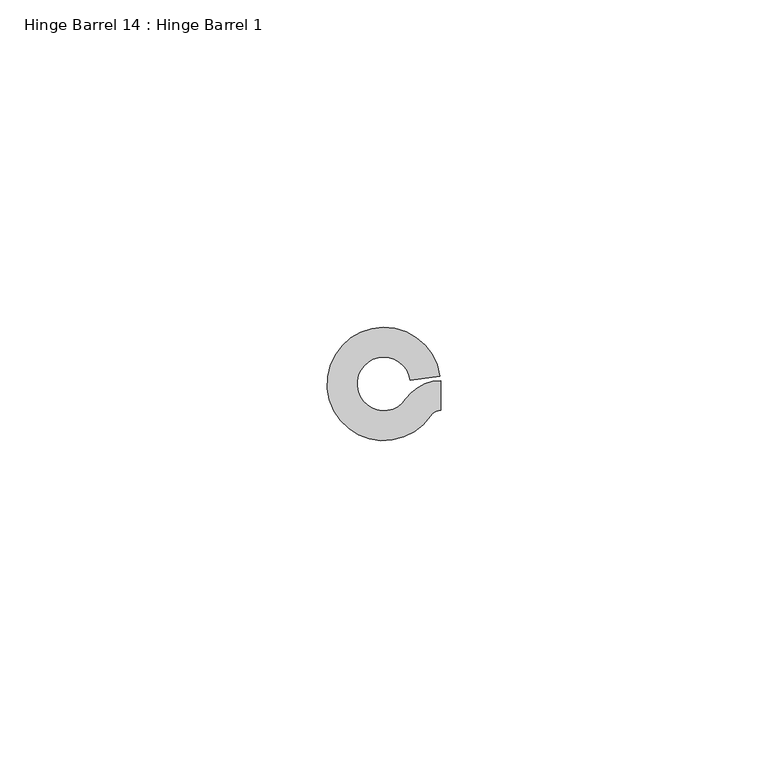
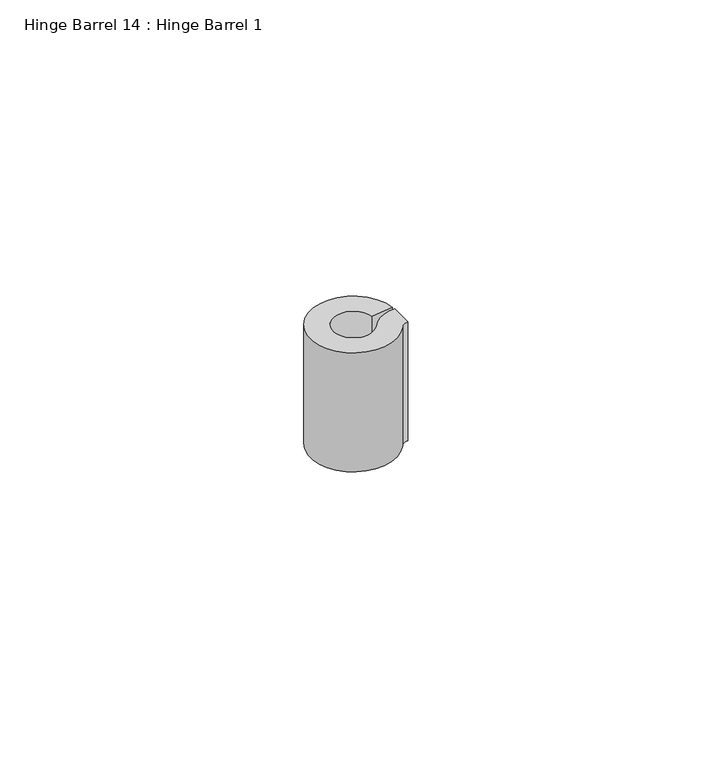
"""IFC4 building model written with IfcOpenShell, lengths in millimetres: proxy geometry, Hinge Barrel 14 : Hinge Barrel 1."""

from ifc_helpers import new_model, si_unit, point, frame, frame_2d, origin, place, context, project, spatial, polyline, circle_curve, trimmed, segment, composite_curve, outline, extrude, source, transform, mapped, element, save


def hinge_barrel_14_hinge_barrel_1_75b3f5ff(model_context):
    return source(origin(), model_context, "Body", "SweptSolid", [
        extrude(outline(composite_curve([segment(trimmed(circle_curve(frame_2d((587327.8245257, -533990.5568067)), 6.4044851), [point((587322.5194669, -533986.9688017))], [point((587327.8245257, -533984.1523216))], False, "CARTESIAN"), True, "CONTINUOUS"), segment(polyline([(587327.8245257, -533984.1523216), (587327.8245257, -533988.7163841)]), True, "CONTINUOUS"), segment(trimmed(circle_curve(frame_2d((587327.8245257, -533990.5568067)), 1.8404226), [point((587327.8245257, -533988.7163841))], [point((587326.3000393, -533989.5257409))], True, "CARTESIAN"), True, "CONTINUOUS"), segment(trimmed(circle_curve(frame_2d((587319.1320739, -533984.6777841)), 8.6534625), [point((587326.3000393, -533989.5257409))], [point((587327.7022899, -533983.4803654))], False, "CARTESIAN"), True, "CONTINUOUS"), segment(polyline([(587327.7022899, -533983.4803654), (587323.1821338, -533984.1119153)]), True, "CONTINUOUS"), segment(trimmed(circle_curve(frame_2d((587319.1320739, -533984.6777841)), 4.0894), [point((587323.1821338, -533984.1119153))], [point((587322.5194669, -533986.9688017))], True, "CARTESIAN"), True, "CONTINUOUS")], self_intersect=False)), frame((0.0, 0.0, 336.55), z_axis=(0.0, 0.0, 1.0), x_axis=(1.0, 0.0, 0.0)), (0.0, 0.0, 1.0), 25.4),
    ])


if __name__ == "__main__":
    model = new_model("IFC4")
    model_context = context("Model", 3, world=origin())
    ifc_project = project(units=[si_unit("LENGTHUNIT", "METRE", prefix="MILLI")], contexts=[model_context])
    site = spatial("IfcSite", under=ifc_project)
    building = spatial("IfcBuilding", under=site)
    placement = place(None, origin())
    hinge_barrel_14_hinge_barrel_1_shape = hinge_barrel_14_hinge_barrel_1_75b3f5ff(model_context)
    element("IfcBuildingElementProxy", 1, Name="Hinge Barrel 14 : Hinge Barrel 1", ObjectType="Hinge Barrel 14 : Hinge Barrel 1", at=placement, inside=building, context=model_context, shape_type="MappedRepresentation", body=[
        mapped(hinge_barrel_14_hinge_barrel_1_shape, transform((0.0, 0.0, 0.0), x_axis=(1.0, 0.0, 0.0), y_axis=(0.0, 1.0, 0.0), z_axis=(0.0, 0.0, 1.0))),
    ])
    save(model, "model.ifc")

# Revit data of these elements
# Element 1 (IfcBuildingElementProxy, "Hinge Barrel 14 : Hinge Barrel 1")
#   Materials on its faces: "6\"X6\" WELD-ON STL BUTT HINGE"
# Materials
#   "6\"X6\" WELD-ON STL BUTT HINGE": class "Metal", colour RGB 189 187 185, transparency 0, Description = "Carbon steel", Cost = 0
